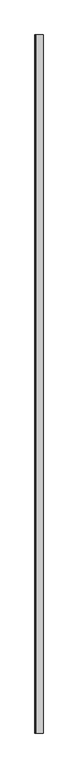
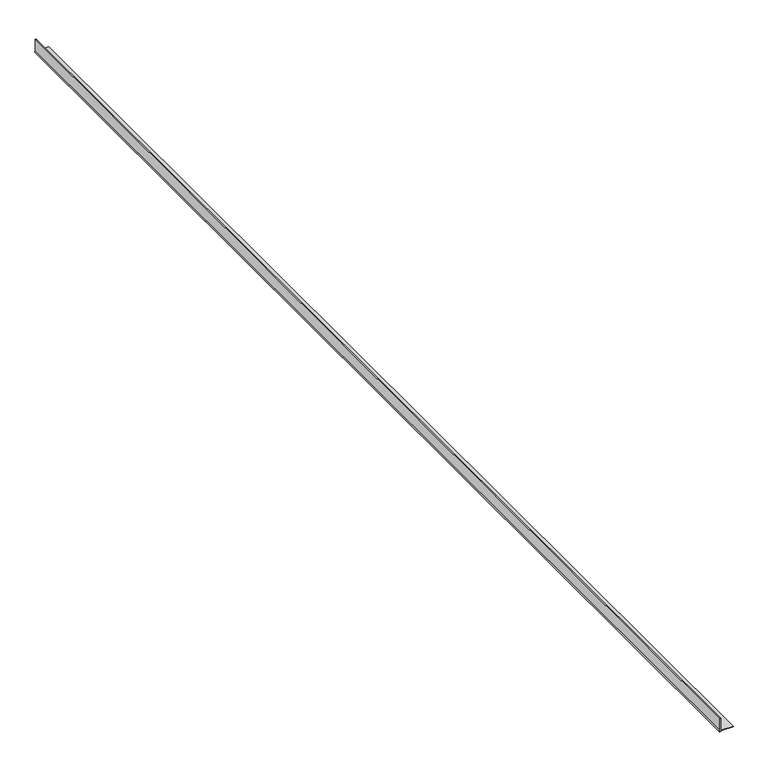
"""IFC4 building model written with IfcOpenShell, lengths in millimetres: proxy geometry, Blocking091 3:Blocking091 17871:303082 : Blocking091 3:Blocking091 17871:303082."""

from ifc_helpers import new_model, si_unit, point, frame, frame_2d, origin, place, context, project, spatial, polyline, circle_curve, trimmed, segment, composite_curve, outline, extrude, source, transform, mapped, element, save


def generic_models_7da3cde2(model_context):
    return source(origin(), model_context, "Body", "SweptSolid", [
        extrude(outline(composite_curve([segment(polyline([(39558.351, 11981.8604648), (39579.5041839, 11981.8604648), (39579.5041839, 11980.5804648), (39558.6202421, 11980.5804648)]), True, "CONTINUOUS"), segment(trimmed(circle_curve(frame_2d((39557.3733211, 11980.9295256)), 1.2948572), [point((39558.6202421, 11980.5804648))], [point((39557.071, 11982.1885956))], False, "CARTESIAN"), True, "CONTINUOUS"), segment(polyline([(39557.071, 11982.1885956), (39557.071, 12003.0136488), (39558.351, 12003.0136488), (39558.351, 11981.8604648)]), True, "CONTINUOUS")], self_intersect=False)), frame((0.0, -3469.6166527, 0.0), z_axis=(0.0, 1.0, 0.0), x_axis=(0.0, 0.0, 1.0)), (0.0, 0.0, 1.0), 2000.0),
    ])


if __name__ == "__main__":
    model = new_model("IFC4")
    model_context = context("Model", 3, world=origin())
    ifc_project = project(units=[si_unit("LENGTHUNIT", "METRE", prefix="MILLI")], contexts=[model_context])
    site = spatial("IfcSite", under=ifc_project)
    building = spatial("IfcBuilding", under=site)
    placement = place(None, origin())
    generic_models_shape = generic_models_7da3cde2(model_context)
    element("IfcBuildingElementProxy", 1, Name="Blocking091 3:Blocking091 17871:303082 : Blocking091 3:Blocking091 17871:303082", ObjectType="Blocking091 3:Blocking091 17871:303082 : Blocking091 3:Blocking091 17871:303082", at=placement, inside=building, context=model_context, shape_type="MappedRepresentation", body=[
        mapped(generic_models_shape, transform((0.0, 0.0, 0.0), x_axis=(1.0, 0.0, 0.0), y_axis=(0.0, 1.0, 0.0), z_axis=(0.0, 0.0, 1.0))),
    ])
    save(model, "model.ifc")

# Revit data of these elements
# Type "Blocking091 3:Blocking091 17871:303082 : Blocking091 3:Blocking091 17871:303082"
#   NameOverride = "Blocking091 3:Blocking091 17871:303082"
#   ObjectTypeOverride = "Blocking091 3:Blocking091 17871"
#   Reference = "Blocking091 17871"
#   Category = "Generic Models"
#   Tag = "303082"
# Element 1 (IfcBuildingElementProxy, "Blocking091 3:Blocking091 17871:303082 : Blocking091 3:Blocking091 17871:303082")
#   Materials on its faces: "CORNER BEAD"
# Materials
#   "CORNER BEAD": class "Unassigned", colour RGB 253 236 176, transparency 0, Cost = 0
